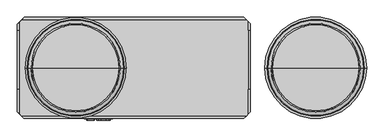
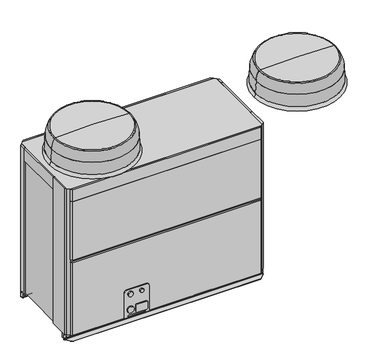
"""IFC4 building model written with IfcOpenShell, lengths in millimetres: proxy geometry, PURY-P168-288_YSJMU_Heat_Recovery_460V : PURY-P192YSJMU-A(-BS)_460V."""

from ifc_helpers import new_model, si_unit, point, frame, frame_2d, origin, place, context, project, spatial, polyline, circle_curve, ellipse_curve, trimmed, segment, composite_curve, outline, extrude, source, transform, mapped, element, save
from ifc_brep_helpers import plane_surface, cylinder_surface, revolved_surface, advanced_brep


def mechanical_equipment_7c6ddfd4(model_context):
    return source(origin(), model_context, "Body", "SolidModel", [
        advanced_brep(
        [(1130.4156536, 0.0, 1550.0000157), (1851.6603464, 0.0, 1550.0000157), (1491.038, 0.0, 1550.0000157), (1156.2569245, 0.0, 1635.7196156), (1825.8190755, 0.0, 1635.7196156), (1165.4260831, 0.0, 1640.2981249), (1816.6499169, 0.0, 1640.2981249), (1491.038, 0.0, 1649.794168)],
        [
            (0, 1, circle_curve(frame((1491.038, 0.0, 1550.0000157), z_axis=(0.0, 0.0, -1.0), x_axis=(1.0, 0.0, 0.0)), 360.6223464)),
            (1, 2),
            (2, 0),
            (1, 0, circle_curve(frame((1491.038, 0.0, 1550.0000157), z_axis=(0.0, 0.0, -1.0), x_axis=(1.0, 0.0, 0.0)), 360.6223464)),
            (3, 4, circle_curve(frame((1491.038, 0.0, 1635.7196156), z_axis=(0.0, 0.0, -1.0), x_axis=(1.0, 0.0, 0.0)), 334.7810755)),
            (4, 1, circle_curve(frame((1667.7568175, 0.0, 1541.3148332), z_axis=(0.0, 1.0, 0.0), x_axis=(1.0, 0.0, 0.0)), 184.1085015)),
            (0, 3, circle_curve(frame((1314.3191825, 0.0, 1541.3148332), z_axis=(0.0, 1.0, 0.0), x_axis=(-1.0, 0.0, 0.0)), 184.1085015)),
            (4, 3, circle_curve(frame((1491.038, 0.0, 1635.7196156), z_axis=(0.0, 0.0, -1.0), x_axis=(1.0, 0.0, 0.0)), 334.7810755)),
            (5, 6, circle_curve(frame((1491.038, 0.0, 1640.2981249), z_axis=(0.0, 0.0, -1.0), x_axis=(1.0, 0.0, 0.0)), 325.6119169)),
            (6, 4, circle_curve(frame((1816.6499169, 0.0, 1628.8275558), z_axis=(0.0, 1.0, 0.0), x_axis=(1.0, 0.0, 0.0)), 11.4705691)),
            (3, 5, circle_curve(frame((1165.4260831, 0.0, 1628.8275558), z_axis=(0.0, 1.0, 0.0), x_axis=(-1.0, 0.0, 0.0)), 11.4705691)),
            (6, 5, circle_curve(frame((1491.038, 0.0, 1640.2981249), z_axis=(0.0, 0.0, -1.0), x_axis=(1.0, 0.0, 0.0)), 325.6119169)),
            (7, 6, circle_curve(frame((1491.038, 0.0, -3937.4433334), z_axis=(0.0, 1.0, 0.0), x_axis=(1.0, 0.0, 0.0)), 5587.2375013)),
            (5, 7, circle_curve(frame((1491.038, 0.0, -3937.4433334), z_axis=(0.0, 1.0, 0.0), x_axis=(-1.0, 0.0, 0.0)), 5587.2375013)),
        ],
        [
            plane_surface(frame((1491.038, 0.0, 1550.0000157), z_axis=(0.0, 0.0, -1.0), x_axis=(1.0, 0.0, 0.0))),
            revolved_surface(trimmed(ellipse_curve(frame((1667.7568175, 0.0, 1541.3148332), z_axis=(0.0, -1.0, 0.0), x_axis=(1.0, 0.0, 0.0)), 184.1085015, 184.1085015), [point((1851.6603464, 0.0, 1550.0000157))], [point((1825.8190755, 0.0, 1635.7196156))], True, "CARTESIAN"), (1491.038, 0.0, 1605.0), (0.0, 0.0, 1.0)),
            revolved_surface(trimmed(ellipse_curve(frame((1816.6499169, 0.0, 1628.8275558), z_axis=(0.0, -1.0, 0.0), x_axis=(1.0, 0.0, 0.0)), 11.4705691, 11.4705691), [point((1825.8190755, 0.0, 1635.7196156))], [point((1816.6499169, 0.0, 1640.2981249))], True, "CARTESIAN"), (1491.038, 0.0, 1605.0), (0.0, 0.0, 1.0)),
            revolved_surface(trimmed(ellipse_curve(frame((1491.038, 0.0, -3937.4433334), z_axis=(0.0, -1.0, 0.0), x_axis=(1.0, 0.0, 0.0)), 5587.2375013, 5587.2375013), [point((1816.6499169, 0.0, 1640.2981249))], [point((1491.038, 0.0, 1649.794168))], True, "CARTESIAN"), (1491.038, 0.0, 1605.0), (0.0, 0.0, 1.0)),
        ],
        [
            (0, [[1, 2, 3]]),
            (0, [[4, -3, -2]]),
            (1, [[5, 6, -1, 7]]),
            (1, [[8, -7, -4, -6]]),
            (2, [[9, 10, -5, 11]]),
            (2, [[12, -11, -8, -10]]),
            (3, [[13, -9, 14]]),
            (3, [[-14, -12, -13]]),
        ],
    ),
        advanced_brep(
        [(1108.9881528, 0.0, 1410.0), (1873.0878472, 0.0, 1410.0), (1491.038, 0.0, 1410.0), (1125.5531583, 0.0, 1438.6914312), (1856.5228417, 0.0, 1438.6914312), (1130.4129453, 0.0, 1550.0000157), (1851.6630547, 0.0, 1550.0000157), (1491.038, 0.0, 1550.0000157)],
        [
            (0, 1, circle_curve(frame((1491.038, 0.0, 1410.0), z_axis=(0.0, 0.0, -1.0), x_axis=(1.0, 0.0, 0.0)), 382.0498472)),
            (1, 2),
            (2, 0),
            (1, 0, circle_curve(frame((1491.038, 0.0, 1410.0), z_axis=(0.0, 0.0, -1.0), x_axis=(1.0, 0.0, 0.0)), 382.0498472)),
            (3, 4, circle_curve(frame((1491.038, 0.0, 1438.6914312), z_axis=(0.0, 0.0, -1.0), x_axis=(1.0, 0.0, 0.0)), 365.4848417)),
            (4, 1, circle_curve(frame((1877.2748091, 0.0, 1431.5449644), z_axis=(0.0, -1.0, 0.0), x_axis=(1.0, 0.0, 0.0)), 21.9480327)),
            (0, 3, circle_curve(frame((1104.8011909, 0.0, 1431.5449644), z_axis=(0.0, -1.0, 0.0), x_axis=(-1.0, 0.0, 0.0)), 21.9480327)),
            (4, 3, circle_curve(frame((1491.038, 0.0, 1438.6914312), z_axis=(0.0, 0.0, -1.0), x_axis=(1.0, 0.0, 0.0)), 365.4848417)),
            (5, 6, circle_curve(frame((1491.038, 0.0, 1550.0000157), z_axis=(0.0, 0.0, -1.0), x_axis=(1.0, 0.0, 0.0)), 360.6250547)),
            (6, 4),
            (3, 5),
            (6, 5, circle_curve(frame((1491.038, 0.0, 1550.0000157), z_axis=(0.0, 0.0, -1.0), x_axis=(1.0, 0.0, 0.0)), 360.6250547)),
            (7, 6),
            (5, 7),
        ],
        [
            plane_surface(frame((1491.038, 0.0, 1410.0), z_axis=(0.0, 0.0, -1.0), x_axis=(1.0, 0.0, 0.0))),
            revolved_surface(trimmed(ellipse_curve(frame((1877.2748091, 0.0, 1431.5449644), z_axis=(0.0, 1.0, 0.0), x_axis=(1.0, 0.0, 0.0)), 21.9480327, 21.9480327), [point((1873.0878472, 0.0, 1410.0))], [point((1856.5228417, 0.0, 1438.6914312))], True, "CARTESIAN"), (1491.038, 0.0, 1470.0), (0.0, 0.0, 1.0)),
            revolved_surface(polyline([(1856.5228417, 0.0, 1438.6914312), (1851.6630547, 0.0, 1550.0000157)]), (1491.038, 0.0, 1470.0), (0.0, 0.0, 1.0)),
            plane_surface(frame((1491.038, 0.0, 1550.0000157), z_axis=(0.0, 0.0, 1.0), x_axis=(1.0, 0.0, 0.0))),
        ],
        [
            (0, [[1, 2, 3]]),
            (0, [[4, -3, -2]]),
            (1, [[5, 6, -1, 7]]),
            (1, [[8, -7, -4, -6]]),
            (2, [[9, 10, -5, 11]]),
            (2, [[12, -11, -8, -10]]),
            (3, [[13, -9, 14]]),
            (3, [[-14, -12, -13]]),
        ],
    ),
        extrude(outline(composite_curve([segment(trimmed(circle_curve(frame_2d((148.5853631, -142.3882489)), 9.9920268), [point((158.5773899, -142.3882489))], [point((148.5853631, -152.3802757))], False, "CARTESIAN"), True, "CONTINUOUS"), segment(polyline([(148.5853631, -152.3802757), (96.5694168, -152.3802757)]), True, "CONTINUOUS"), segment(trimmed(circle_curve(frame_2d((96.5694168, -142.3882489)), 9.9920268), [point((96.5694168, -152.3802757))], [point((86.5773899, -142.3882489))], False, "CARTESIAN"), True, "CONTINUOUS"), segment(polyline([(86.5773899, -142.3882489), (86.5773899, -60.3723026)]), True, "CONTINUOUS"), segment(trimmed(circle_curve(frame_2d((96.5694168, -60.3723026)), 9.9920268), [point((86.5773899, -60.3723026))], [point((96.5694168, -50.3802757))], False, "CARTESIAN"), True, "CONTINUOUS"), segment(polyline([(96.5694168, -50.3802757), (148.5853631, -50.3802757)]), True, "CONTINUOUS"), segment(trimmed(circle_curve(frame_2d((148.5853631, -60.3723026)), 9.9920268), [point((148.5853631, -50.3802757))], [point((158.5773899, -60.3723026))], False, "CARTESIAN"), True, "CONTINUOUS"), segment(polyline([(158.5773899, -60.3723026), (158.5773899, -142.3882489)]), True, "CONTINUOUS")], self_intersect=False)), frame((0.0, -397.2710787, 0.0), z_axis=(0.0, 1.0, 0.0), x_axis=(0.0, 0.0, 1.0)), (0.0, 0.0, 1.0), 12.5),
        extrude(outline(composite_curve([segment(trimmed(circle_curve(frame_2d((292.0295314, -55.1286698)), 21.9704686), [point((292.0295314, -33.1582012))], [point((314.0, -55.1286698))], False, "CARTESIAN"), True, "CONTINUOUS"), segment(polyline([(314.0, -55.1286698), (314.0, -226.9915314)]), True, "CONTINUOUS"), segment(trimmed(circle_curve(frame_2d((292.0295314, -226.9915314)), 21.9704686), [point((314.0, -226.9915314))], [point((292.0295314, -248.962))], False, "CARTESIAN"), True, "CONTINUOUS"), segment(polyline([(292.0295314, -248.962), (54.0, -248.962), (54.0, -33.1582012), (292.0295314, -33.1582012)]), True, "CONTINUOUS")], self_intersect=False), holes=[composite_curve([segment(trimmed(circle_curve(frame_2d((66.0219764, -74.4132816)), 7.4940201), [point((73.5159966, -74.4132816))], [point((58.5279563, -74.4132816))], True, "CARTESIAN"), True, "CONTINUOUS"), segment(polyline([(58.5279563, -74.4132816), (58.5279563, -209.3056439)]), True, "CONTINUOUS"), segment(trimmed(circle_curve(frame_2d((66.0219764, -209.3056439)), 7.4940201), [point((58.5279563, -209.3056439))], [point((73.5159966, -209.3056439))], True, "CARTESIAN"), True, "CONTINUOUS"), segment(polyline([(73.5159966, -209.3056439), (73.5159966, -74.4132816)]), True, "CONTINUOUS")], self_intersect=False)]), frame((0.0, -384.7710787, 0.0), z_axis=(0.0, 1.0, 0.0), x_axis=(0.0, 0.0, 1.0)), (0.0, 0.0, 1.0), 4.7710787),
        extrude(outline(composite_curve([segment(trimmed(circle_curve(frame_2d((272.5206481, -199.3802757)), 22.225), [point((272.5206481, -221.6052757))], [point((272.5206481, -177.1552757))], False, "CARTESIAN"), True, "CONTINUOUS"), segment(trimmed(circle_curve(frame_2d((272.5206481, -199.3802757)), 22.225), [point((272.5206481, -177.1552757))], [point((272.5206481, -221.6052757))], False, "CARTESIAN"), True, "CONTINUOUS")], self_intersect=False)), frame((0.0, -397.2710787, 0.0), z_axis=(0.0, 1.0, 0.0), x_axis=(0.0, 0.0, 1.0)), (0.0, 0.0, 1.0), 12.5),
        extrude(outline(composite_curve([segment(trimmed(circle_curve(frame_2d((272.5206481, -101.3802757)), 17.0), [point((272.5206481, -118.3802757))], [point((272.5206481, -84.3802757))], False, "CARTESIAN"), True, "CONTINUOUS"), segment(trimmed(circle_curve(frame_2d((272.5206481, -101.3802757)), 17.0), [point((272.5206481, -84.3802757))], [point((272.5206481, -118.3802757))], False, "CARTESIAN"), True, "CONTINUOUS")], self_intersect=False)), frame((0.0, -397.2710787, 0.0), z_axis=(0.0, 1.0, 0.0), x_axis=(0.0, 0.0, 1.0)), (0.0, 0.0, 1.0), 12.5),
        extrude(outline(composite_curve([segment(trimmed(circle_curve(frame_2d((127.8409633, -199.3802757)), 28.575), [point((127.8409633, -227.9552757))], [point((127.8409633, -170.8052757))], False, "CARTESIAN"), True, "CONTINUOUS"), segment(trimmed(circle_curve(frame_2d((127.8409633, -199.3802757)), 28.575), [point((127.8409633, -170.8052757))], [point((127.8409633, -227.9552757))], False, "CARTESIAN"), True, "CONTINUOUS")], self_intersect=False)), frame((0.0, -397.2710787, 0.0), z_axis=(0.0, 1.0, 0.0), x_axis=(0.0, 0.0, 1.0)), (0.0, 0.0, 1.0), 12.5),
        extrude(outline(polyline([(1001.038, 284.0), (985.038, 284.0), (985.038, 346.9999976), (1001.038, 330.9999976), (1001.038, 284.0)])), frame((0.0, 0.0, 54.0), z_axis=(0.0, 0.0, 1.0), x_axis=(1.0, 0.0, 0.0)), (0.0, 0.0, 1.0), 1356.0),
        extrude(outline(polyline([(985.038, -164.0), (1001.038, -164.0), (1001.038, -331.000002), (985.038, -347.000002), (985.038, -164.0)])), frame((0.0, 0.0, 54.0), z_axis=(0.0, 0.0, 1.0), x_axis=(1.0, 0.0, 0.0)), (0.0, 0.0, 1.0), 1356.0),
        extrude(outline(polyline([(932.5551598, 364.0), (932.5551598, 380.0), (952.0379976, 380.0), (968.0379976, 364.0), (932.5551598, 364.0)])), frame((0.0, 0.0, 54.0), z_axis=(0.0, 0.0, 1.0), x_axis=(1.0, 0.0, 0.0)), (0.0, 0.0, 1.0), 1245.8),
        extrude(outline(polyline([(-670.129169, 380.0), (-670.129169, 364.0), (-714.5495072, 364.0), (-698.5495072, 380.0), (-670.129169, 380.0)])), frame((0.0, 0.0, 54.0), z_axis=(0.0, 0.0, 1.0), x_axis=(1.0, 0.0, 0.0)), (0.0, 0.0, 1.0), 1245.8),
        extrude(outline(polyline([(968.0379976, 364.0), (-714.5495072, 364.0), (-698.5495072, 380.0), (952.0379976, 380.0), (968.0379976, 364.0)])), frame((0.0, 0.0, 1299.8), z_axis=(0.0, 0.0, 1.0), x_axis=(1.0, 0.0, 0.0)), (0.0, 0.0, 1.0), 110.2),
        extrude(outline(polyline([(952.038002, -380.0), (-699.9620129, -380.0), (-715.9620129, -364.0), (968.038002, -364.0), (952.038002, -380.0)])), frame((0.0, 0.0, 1299.8), z_axis=(0.0, 0.0, 1.0), x_axis=(1.0, 0.0, 0.0)), (0.0, 0.0, 1.0), 110.2),
        extrude(outline(polyline([(-715.9620129, -364.0), (968.038002, -364.0), (952.038002, -380.0), (-699.9620129, -380.0), (-715.9620129, -364.0)])), frame((0.0, 0.0, 755.5000076), z_axis=(0.0, 0.0, 1.0), x_axis=(1.0, 0.0, 0.0)), (0.0, 0.0, 1.0), 544.2999924),
        extrude(outline(polyline([(-732.962, -347.0000129), (-732.962, 345.5875072), (-714.5495072, 364.0), (968.0379976, 364.0), (985.038, 346.9999976), (985.038, -347.000002), (968.038002, -364.0), (-715.9620129, -364.0), (-732.962, -347.0000129)])), frame((0.0, 0.0, 54.0), z_axis=(0.0, 0.0, 1.0), x_axis=(1.0, 0.0, 0.0)), (0.0, 0.0, 1.0), 1356.0),
        extrude(outline(polyline([(-732.962, 284.0), (-748.962, 284.0), (-748.962, 329.5875072), (-732.962, 345.5875072), (-732.962, 284.0)])), frame((0.0, 0.0, 54.0), z_axis=(0.0, 0.0, 1.0), x_axis=(1.0, 0.0, 0.0)), (0.0, 0.0, 1.0), 1356.0),
        extrude(outline(polyline([(-748.962, -164.0), (-732.962, -164.0), (-732.962, -347.0000129), (-748.962, -331.0000129), (-748.962, -164.0)])), frame((0.0, 0.0, 54.0), z_axis=(0.0, 0.0, 1.0), x_axis=(1.0, 0.0, 0.0)), (0.0, 0.0, 1.0), 1356.0),
        extrude(outline(polyline([(-715.9620129, -364.0), (968.038002, -364.0), (952.038002, -380.0), (-699.9620129, -380.0), (-715.9620129, -364.0)])), frame((0.0, 0.0, 54.0), z_axis=(0.0, 0.0, 1.0), x_axis=(1.0, 0.0, 0.0)), (0.0, 0.0, 1.0), 678.5000074),
        extrude(outline(polyline([(161.038, 364.0), (161.038, 380.0), (932.5551598, 380.0), (932.5551598, 364.0), (161.038, 364.0)])), frame((0.0, 0.0, 54.0), z_axis=(0.0, 0.0, 1.0), x_axis=(1.0, 0.0, 0.0)), (0.0, 0.0, 1.0), 1245.8),
        extrude(outline(polyline([(161.038, 339.0), (141.038, 339.0), (141.038, 380.0), (161.038, 380.0), (161.038, 339.0)])), frame((0.0, 0.0, 54.0), z_axis=(0.0, 0.0, 1.0), x_axis=(1.0, 0.0, 0.0)), (0.0, 0.0, 1.0), 1245.8),
        extrude(outline(polyline([(111.038, 339.0), (91.038, 339.0), (91.038, 380.0), (111.038, 380.0), (111.038, 339.0)])), frame((0.0, 0.0, 54.0), z_axis=(0.0, 0.0, 1.0), x_axis=(1.0, 0.0, 0.0)), (0.0, 0.0, 1.0), 1245.8),
        advanced_brep(
        [(-672.0843464, 0.0, 1550.0000157), (49.1603464, 0.0, 1550.0000157), (-311.462, 0.0, 1550.0000157), (-646.2430755, 0.0, 1635.7196156), (23.3190755, 0.0, 1635.7196156), (-637.0739169, 0.0, 1640.2981249), (14.1499169, 0.0, 1640.2981249), (-311.462, 0.0, 1649.7941679)],
        [
            (0, 1, circle_curve(frame((-311.462, 0.0, 1550.0000157), z_axis=(0.0, 0.0, -1.0), x_axis=(1.0, 0.0, 0.0)), 360.6223464)),
            (1, 2),
            (2, 0),
            (1, 0, circle_curve(frame((-311.462, 0.0, 1550.0000157), z_axis=(0.0, 0.0, -1.0), x_axis=(1.0, 0.0, 0.0)), 360.6223464)),
            (3, 4, circle_curve(frame((-311.462, 0.0, 1635.7196156), z_axis=(0.0, 0.0, -1.0), x_axis=(1.0, 0.0, 0.0)), 334.7810755)),
            (4, 1, circle_curve(frame((-134.7431825, 0.0, 1541.3148332), z_axis=(0.0, 1.0, 0.0), x_axis=(1.0, 0.0, 0.0)), 184.1085015)),
            (0, 3, circle_curve(frame((-488.1808175, 0.0, 1541.3148332), z_axis=(0.0, 1.0, 0.0), x_axis=(-1.0, 0.0, 0.0)), 184.1085015)),
            (4, 3, circle_curve(frame((-311.462, 0.0, 1635.7196156), z_axis=(0.0, 0.0, -1.0), x_axis=(1.0, 0.0, 0.0)), 334.7810755)),
            (5, 6, circle_curve(frame((-311.462, 0.0, 1640.2981249), z_axis=(0.0, 0.0, -1.0), x_axis=(1.0, 0.0, 0.0)), 325.6119169)),
            (6, 4, circle_curve(frame((14.1499169, 0.0, 1628.8275558), z_axis=(0.0, 1.0, 0.0), x_axis=(1.0, 0.0, 0.0)), 11.4705691)),
            (3, 5, circle_curve(frame((-637.0739169, 0.0, 1628.8275558), z_axis=(0.0, 1.0, 0.0), x_axis=(-1.0, 0.0, 0.0)), 11.4705691)),
            (6, 5, circle_curve(frame((-311.462, 0.0, 1640.2981249), z_axis=(0.0, 0.0, -1.0), x_axis=(1.0, 0.0, 0.0)), 325.6119169)),
            (7, 6, circle_curve(frame((-311.462, 0.0, -3937.4433334), z_axis=(0.0, 1.0, 0.0), x_axis=(1.0, 0.0, 0.0)), 5587.2375013)),
            (5, 7, circle_curve(frame((-311.462, 0.0, -3937.4433334), z_axis=(0.0, 1.0, 0.0), x_axis=(-1.0, 0.0, 0.0)), 5587.2375013)),
        ],
        [
            plane_surface(frame((-311.462, 0.0, 1550.0000157), z_axis=(0.0, 0.0, -1.0), x_axis=(1.0, 0.0, 0.0))),
            revolved_surface(trimmed(ellipse_curve(frame((-134.7431825, 0.0, 1541.3148332), z_axis=(0.0, -1.0, 0.0), x_axis=(1.0, 0.0, 0.0)), 184.1085015, 184.1085015), [point((49.1603464, 0.0, 1550.0000157))], [point((23.3190755, 0.0, 1635.7196156))], True, "CARTESIAN"), (-311.462, 0.0, 1605.0), (0.0, 0.0, 1.0)),
            revolved_surface(trimmed(ellipse_curve(frame((14.1499169, 0.0, 1628.8275558), z_axis=(0.0, -1.0, 0.0), x_axis=(1.0, 0.0, 0.0)), 11.4705691, 11.4705691), [point((23.3190755, 0.0, 1635.7196156))], [point((14.1499169, 0.0, 1640.2981249))], True, "CARTESIAN"), (-311.462, 0.0, 1605.0), (0.0, 0.0, 1.0)),
            revolved_surface(trimmed(ellipse_curve(frame((-311.462, 0.0, -3937.4433334), z_axis=(0.0, -1.0, 0.0), x_axis=(1.0, 0.0, 0.0)), 5587.2375013, 5587.2375013), [point((14.1499169, 0.0, 1640.2981249))], [point((-311.462, 0.0, 1649.7941679))], True, "CARTESIAN"), (-311.462, 0.0, 1605.0), (0.0, 0.0, 1.0)),
        ],
        [
            (0, [[1, 2, 3]]),
            (0, [[4, -3, -2]]),
            (1, [[5, 6, -1, 7]]),
            (1, [[8, -7, -4, -6]]),
            (2, [[9, 10, -5, 11]]),
            (2, [[12, -11, -8, -10]]),
            (3, [[13, -9, 14]]),
            (3, [[-14, -12, -13]]),
        ],
    ),
        advanced_brep(
        [(-693.5118472, 0.0, 1410.0), (70.5878472, 0.0, 1410.0), (-311.462, 0.0, 1410.0), (-676.9468417, 0.0, 1438.6914312), (54.0228417, 0.0, 1438.6914312), (-672.0870547, 0.0, 1550.0000157), (49.1630547, 0.0, 1550.0000157), (-311.462, 0.0, 1550.0000157)],
        [
            (0, 1, circle_curve(frame((-311.462, 0.0, 1410.0), z_axis=(0.0, 0.0, -1.0), x_axis=(1.0, 0.0, 0.0)), 382.0498472)),
            (1, 2),
            (2, 0),
            (1, 0, circle_curve(frame((-311.462, 0.0, 1410.0), z_axis=(0.0, 0.0, -1.0), x_axis=(1.0, 0.0, 0.0)), 382.0498472)),
            (3, 4, circle_curve(frame((-311.462, 0.0, 1438.6914312), z_axis=(0.0, 0.0, -1.0), x_axis=(1.0, 0.0, 0.0)), 365.4848417)),
            (4, 1, circle_curve(frame((74.7748091, 0.0, 1431.5449644), z_axis=(0.0, -1.0, 0.0), x_axis=(1.0, 0.0, 0.0)), 21.9480327)),
            (0, 3, circle_curve(frame((-697.6988091, 0.0, 1431.5449644), z_axis=(0.0, -1.0, 0.0), x_axis=(-1.0, 0.0, 0.0)), 21.9480327)),
            (4, 3, circle_curve(frame((-311.462, 0.0, 1438.6914312), z_axis=(0.0, 0.0, -1.0), x_axis=(1.0, 0.0, 0.0)), 365.4848417)),
            (5, 6, circle_curve(frame((-311.462, 0.0, 1550.0000157), z_axis=(0.0, 0.0, -1.0), x_axis=(1.0, 0.0, 0.0)), 360.6250547)),
            (6, 4),
            (3, 5),
            (6, 5, circle_curve(frame((-311.462, 0.0, 1550.0000157), z_axis=(0.0, 0.0, -1.0), x_axis=(1.0, 0.0, 0.0)), 360.6250547)),
            (7, 6),
            (5, 7),
        ],
        [
            plane_surface(frame((-311.462, 0.0, 1410.0), z_axis=(0.0, 0.0, -1.0), x_axis=(1.0, 0.0, 0.0))),
            revolved_surface(trimmed(ellipse_curve(frame((74.7748091, 0.0, 1431.5449644), z_axis=(0.0, 1.0, 0.0), x_axis=(1.0, 0.0, 0.0)), 21.9480327, 21.9480327), [point((70.5878472, 0.0, 1410.0))], [point((54.0228417, 0.0, 1438.6914312))], True, "CARTESIAN"), (-311.462, 0.0, 1470.0), (0.0, 0.0, 1.0)),
            revolved_surface(polyline([(54.0228417, 0.0, 1438.6914312), (49.1630547, 0.0, 1550.0000157)]), (-311.462, 0.0, 1470.0), (0.0, 0.0, 1.0)),
            plane_surface(frame((-311.462, 0.0, 1550.0000157), z_axis=(0.0, 0.0, 1.0), x_axis=(1.0, 0.0, 0.0))),
        ],
        [
            (0, [[1, 2, 3]]),
            (0, [[4, -3, -2]]),
            (1, [[5, 6, -1, 7]]),
            (1, [[8, -7, -4, -6]]),
            (2, [[9, 10, -5, 11]]),
            (2, [[12, -11, -8, -10]]),
            (3, [[13, -9, 14]]),
            (3, [[-14, -12, -13]]),
        ],
    ),
        extrude(outline(polyline([(-670.129169, 364.0), (-670.129169, 380.0), (91.038, 380.0), (91.038, 364.0), (-670.129169, 364.0)])), frame((0.0, 0.0, 54.0), z_axis=(0.0, 0.0, 1.0), x_axis=(1.0, 0.0, 0.0)), (0.0, 0.0, 1.0), 1245.8),
        advanced_brep(
        [(1001.038, 330.9999976, 2.3), (1001.038, 330.9999976, 0.0), (952.0379976, 380.0, 0.0), (952.0379976, 380.0, 2.3), (-748.962, 329.5875072, 0.0), (-748.962, 329.5875072, 2.3), (-698.5495072, 380.0, 2.3), (-698.5495072, 380.0, 0.0), (1001.038, 329.5875072, 2.3), (1001.038, 324.5875071, 7.3000001), (1001.038, 324.5875071, 11.7000001), (1001.038, 325.5875071, 12.7000001), (1001.038, 327.5875072, 12.7000001), (1001.038, 327.5875072, 47.3000005), (1001.038, 325.5875071, 47.3000005), (1001.038, 324.5875071, 48.3000005), (1001.038, 324.5875071, 50.0000004), (1001.038, 320.5875077, 53.9999997), (1001.038, 299.5875069, 53.9999997), (1001.038, 299.5875069, 14.0000001), (1001.038, 304.5875069, 9.0000001), (1001.038, 322.2875071, 9.0000001), (1001.038, 322.2875071, 7.3000001), (1001.038, 329.5875072, 0.0), (-748.962, 322.2875071, 7.3000001), (-748.962, 322.2875071, 9.0000001), (-748.962, 304.5875069, 9.0000001), (-748.962, 299.5875069, 14.0000001), (-748.962, 299.5875069, 53.9999997), (-748.962, 320.5875077, 53.9999997), (-748.962, 324.5875071, 50.0000004), (-748.962, 324.5875071, 48.3000005), (-748.962, 325.5875071, 47.3000005), (-748.962, 327.5875072, 47.3000005), (-748.962, 327.5875072, 12.7000001), (-748.962, 325.5875071, 12.7000001), (-748.962, 324.5875071, 11.7000001), (-748.962, 324.5875071, 7.3000001), (972.288009, 327.5875072, 45.0000005), (930.7880086, 327.5875072, 45.0000005), (924.7880085, 327.5875072, 39.0000004), (924.7880085, 327.5875072, 21.0000002), (930.7880086, 327.5875072, 15.0000002), (972.288009, 327.5875072, 15.0000002), (978.2880091, 327.5875072, 21.0000002), (978.2880091, 327.5875072, 39.0000004), (-720.9619997, 327.5875072, 45.0000005), (-726.9619998, 327.5875072, 39.0000004), (-726.9619998, 327.5875072, 21.0000002), (-720.9619997, 327.5875072, 15.0000002), (-679.4619993, 327.5875072, 15.0000002), (-673.4619992, 327.5875072, 21.0000002), (-673.4619992, 327.5875072, 39.0000004), (-679.4619993, 327.5875072, 45.0000005), (930.7880086, 299.5875069, 45.0000005), (972.288009, 299.5875069, 45.0000005), (978.2880091, 299.5875069, 39.0000004), (978.2880091, 299.5875069, 21.0000002), (972.288009, 299.5875069, 15.0000002), (930.7880086, 299.5875069, 15.0000002), (924.7880085, 299.5875069, 21.0000002), (924.7880085, 299.5875069, 39.0000004), (-726.9619998, 299.5875069, 39.0000004), (-720.9619997, 299.5875069, 45.0000005), (-679.4619993, 299.5875069, 45.0000005), (-673.4619992, 299.5875069, 39.0000004), (-673.4619992, 299.5875069, 21.0000002), (-679.4619993, 299.5875069, 15.0000002), (-720.9619997, 299.5875069, 15.0000002), (-726.9619998, 299.5875069, 21.0000002)],
        [
            (0, 1),
            (1, 2),
            (2, 3),
            (3, 0),
            (4, 5),
            (5, 6),
            (6, 7),
            (7, 4),
            (8, 9, circle_curve(frame((1001.038, 329.5875072, 7.3000001), z_axis=(-1.0, 0.0, 0.0), x_axis=(0.0, 1.0, 0.0)), 5.0000001)),
            (9, 10),
            (10, 11, circle_curve(frame((1001.038, 325.5875071, 11.7000001), z_axis=(-1.0, 0.0, 0.0), x_axis=(0.0, 1.0, 0.0)), 1.0)),
            (11, 12),
            (12, 13),
            (13, 14),
            (14, 15, circle_curve(frame((1001.038, 325.5875071, 48.3000005), z_axis=(-1.0, 0.0, 0.0), x_axis=(0.0, 1.0, 0.0)), 1.0)),
            (15, 16),
            (16, 17, circle_curve(frame((1001.038, 320.5875077, 50.0000004), z_axis=(1.0, 0.0, 0.0), x_axis=(0.0, 1.0, 0.0)), 3.9999994)),
            (17, 18),
            (18, 19),
            (19, 20, circle_curve(frame((1001.038, 304.5875069, 14.0000001), z_axis=(1.0, 0.0, 0.0), x_axis=(0.0, 1.0, 0.0)), 5.0000001)),
            (20, 21),
            (21, 22),
            (22, 23, circle_curve(frame((1001.038, 329.5875072, 7.3000001), z_axis=(1.0, 0.0, 0.0), x_axis=(0.0, 1.0, 0.0)), 7.3000001)),
            (23, 1),
            (0, 8),
            (4, 24, circle_curve(frame((-748.962, 329.5875072, 7.3000001), z_axis=(-1.0, 0.0, 0.0), x_axis=(0.0, 1.0, 0.0)), 7.3000001)),
            (24, 25),
            (25, 26),
            (26, 27, circle_curve(frame((-748.962, 304.5875069, 14.0000001), z_axis=(-1.0, 0.0, 0.0), x_axis=(0.0, 1.0, 0.0)), 5.0000001)),
            (27, 28),
            (28, 29),
            (29, 30, circle_curve(frame((-748.962, 320.5875077, 50.0000004), z_axis=(-1.0, 0.0, 0.0), x_axis=(0.0, 1.0, 0.0)), 3.9999994)),
            (30, 31),
            (31, 32, circle_curve(frame((-748.962, 325.5875071, 48.3000005), z_axis=(1.0, 0.0, 0.0), x_axis=(0.0, 1.0, 0.0)), 1.0)),
            (32, 33),
            (33, 34),
            (34, 35),
            (35, 36, circle_curve(frame((-748.962, 325.5875071, 11.7000001), z_axis=(1.0, 0.0, 0.0), x_axis=(0.0, 1.0, 0.0)), 1.0)),
            (36, 37),
            (37, 5, circle_curve(frame((-748.962, 329.5875072, 7.3000001), z_axis=(1.0, 0.0, 0.0), x_axis=(0.0, 1.0, 0.0)), 5.0000001)),
            (8, 5),
            (37, 9),
            (36, 10),
            (35, 11),
            (34, 12),
            (33, 13),
            (38, 39),
            (39, 40, circle_curve(frame((930.7880086, 327.5875072, 39.0000004), z_axis=(0.0, -1.0, 0.0), x_axis=(1.0, 0.0, 0.0)), 6.0000001)),
            (40, 41),
            (41, 42, circle_curve(frame((930.7880086, 327.5875072, 21.0000002), z_axis=(0.0, -1.0, 0.0), x_axis=(1.0, 0.0, 0.0)), 6.0000001)),
            (42, 43),
            (43, 44, circle_curve(frame((972.288009, 327.5875072, 21.0000002), z_axis=(0.0, -1.0, 0.0), x_axis=(1.0, 0.0, 0.0)), 6.0000001)),
            (44, 45),
            (45, 38, circle_curve(frame((972.288009, 327.5875072, 39.0000004), z_axis=(0.0, -1.0, 0.0), x_axis=(1.0, 0.0, 0.0)), 6.0000001)),
            (46, 47, circle_curve(frame((-720.9619997, 327.5875072, 39.0000004), z_axis=(0.0, -1.0, 0.0), x_axis=(1.0, 0.0, 0.0)), 6.0000001)),
            (47, 48),
            (48, 49, circle_curve(frame((-720.9619997, 327.5875072, 21.0000002), z_axis=(0.0, -1.0, 0.0), x_axis=(1.0, 0.0, 0.0)), 6.0000001)),
            (49, 50),
            (50, 51, circle_curve(frame((-679.4619993, 327.5875072, 21.0000002), z_axis=(0.0, -1.0, 0.0), x_axis=(1.0, 0.0, 0.0)), 6.0000001)),
            (51, 52),
            (52, 53, circle_curve(frame((-679.4619993, 327.5875072, 39.0000004), z_axis=(0.0, -1.0, 0.0), x_axis=(1.0, 0.0, 0.0)), 6.0000001)),
            (53, 46),
            (32, 14),
            (31, 15),
            (30, 16),
            (29, 17),
            (28, 18),
            (27, 19),
            (54, 55),
            (55, 56, circle_curve(frame((972.288009, 299.5875069, 39.0000004), z_axis=(0.0, 1.0, 0.0), x_axis=(1.0, 0.0, 0.0)), 6.0000001)),
            (56, 57),
            (57, 58, circle_curve(frame((972.288009, 299.5875069, 21.0000002), z_axis=(0.0, 1.0, 0.0), x_axis=(1.0, 0.0, 0.0)), 6.0000001)),
            (58, 59),
            (59, 60, circle_curve(frame((930.7880086, 299.5875069, 21.0000002), z_axis=(0.0, 1.0, 0.0), x_axis=(1.0, 0.0, 0.0)), 6.0000001)),
            (60, 61),
            (61, 54, circle_curve(frame((930.7880086, 299.5875069, 39.0000004), z_axis=(0.0, 1.0, 0.0), x_axis=(1.0, 0.0, 0.0)), 6.0000001)),
            (62, 63, circle_curve(frame((-720.9619997, 299.5875069, 39.0000004), z_axis=(0.0, 1.0, 0.0), x_axis=(1.0, 0.0, 0.0)), 6.0000001)),
            (63, 64),
            (64, 65, circle_curve(frame((-679.4619993, 299.5875069, 39.0000004), z_axis=(0.0, 1.0, 0.0), x_axis=(1.0, 0.0, 0.0)), 6.0000001)),
            (65, 66),
            (66, 67, circle_curve(frame((-679.4619993, 299.5875069, 21.0000002), z_axis=(0.0, 1.0, 0.0), x_axis=(1.0, 0.0, 0.0)), 6.0000001)),
            (67, 68),
            (68, 69, circle_curve(frame((-720.9619997, 299.5875069, 21.0000002), z_axis=(0.0, 1.0, 0.0), x_axis=(1.0, 0.0, 0.0)), 6.0000001)),
            (69, 62),
            (26, 20),
            (25, 21),
            (24, 22),
            (4, 23),
            (7, 2),
            (6, 3),
            (38, 55),
            (54, 39),
            (61, 40),
            (60, 41),
            (59, 42),
            (58, 43),
            (57, 44),
            (56, 45),
            (46, 63),
            (62, 47),
            (69, 48),
            (68, 49),
            (67, 50),
            (66, 51),
            (65, 52),
            (64, 53),
        ],
        [
            plane_surface(frame((952.0379976, 380.0, 1410.0), z_axis=(0.7071067811865354, 0.7071067811865598, 0.0), x_axis=(0.0, 0.0, -1.0))),
            plane_surface(frame((-748.962, 329.5875072, 1410.0), z_axis=(-0.707106781186156, 0.7071067811869391, 0.0), x_axis=(0.0, 0.0, -1.0))),
            plane_surface(frame((1001.038, 334.5875072, 7.3000001), z_axis=(1.0, 0.0, 0.0), x_axis=(0.0, 0.0, -1.0))),
            plane_surface(frame((-748.962, 334.5875072, 7.3000001), z_axis=(-1.0, 0.0, 0.0), x_axis=(0.0, 0.0, 1.0))),
            revolved_surface(polyline([(-748.962, 334.5875073, 7.3000001), (1001.038, 334.5875073, 7.3000001)]), (-748.962, 329.5875072, 7.3000001), (-1.0, 0.0, 0.0)),
            plane_surface(frame((1001.038, 324.5875071, 7.3000001), z_axis=(0.0, 1.0, 0.0), x_axis=(-1.0, 0.0, 0.0))),
            revolved_surface(polyline([(-748.962, 326.5875071, 11.7000001), (1001.038, 326.5875071, 11.7000001)]), (-748.962, 325.5875071, 11.7000001), (-1.0, 0.0, 0.0)),
            plane_surface(frame((1001.038, 325.5875071, 12.7000001), z_axis=(0.0, 0.0, -1.0), x_axis=(-1.0, 0.0, 0.0))),
            plane_surface(frame((1001.038, 327.5875072, 12.7000001), z_axis=(0.0, 1.0, 0.0), x_axis=(-1.0, 0.0, 0.0))),
            plane_surface(frame((1001.038, 327.5875072, 47.3000005), z_axis=(0.0, 0.0, 1.0), x_axis=(-1.0, 0.0, 0.0))),
            revolved_surface(polyline([(-748.962, 326.5875071, 48.3000005), (1001.038, 326.5875071, 48.3000005)]), (-748.962, 325.5875071, 48.3000005), (-1.0, 0.0, 0.0)),
            plane_surface(frame((1001.038, 324.5875071, 48.3000005), z_axis=(0.0, 1.0, 0.0), x_axis=(-1.0, 0.0, 0.0))),
            cylinder_surface(frame((-748.962, 320.5875077, 50.0000004), z_axis=(1.0, 0.0, 0.0), x_axis=(0.0, 1.0, 0.0)), 3.9999994),
            plane_surface(frame((1001.038, 320.5875077, 53.9999997), z_axis=(0.0, 0.0, 1.0), x_axis=(-1.0, 0.0, 0.0))),
            plane_surface(frame((1001.038, 299.5875069, 53.9999997), z_axis=(0.0, -1.0, 0.0), x_axis=(-1.0, 0.0, 0.0))),
            cylinder_surface(frame((-748.962, 304.5875069, 14.0000001), z_axis=(1.0, 0.0, 0.0), x_axis=(0.0, 1.0, 0.0)), 5.0000001),
            plane_surface(frame((1001.038, 304.5875069, 9.0000001), z_axis=(0.0, 0.0, -1.0), x_axis=(-1.0, 0.0, 0.0))),
            plane_surface(frame((1001.038, 322.2875071, 9.0000001), z_axis=(0.0, -1.0, 0.0), x_axis=(-1.0, 0.0, 0.0))),
            cylinder_surface(frame((-748.962, 329.5875072, 7.3000001), z_axis=(1.0, 0.0, 0.0), x_axis=(0.0, 1.0, 0.0)), 7.3000001),
            plane_surface(frame((1001.038, 329.5875072, 0.0), z_axis=(0.0, 0.0, -1.0), x_axis=(-1.0, 0.0, 0.0))),
            plane_surface(frame((1001.038, 380.0, 0.0), z_axis=(0.0, 1.0, 0.0), x_axis=(-1.0, 0.0, 0.0))),
            plane_surface(frame((1001.038, 380.0, 2.3), z_axis=(0.0, 0.0, 1.0), x_axis=(-1.0, 0.0, 0.0))),
            plane_surface(frame((972.288009, -339.0, 45.0000005), z_axis=(0.0, 0.0, -1.0), x_axis=(0.0, 1.0, 0.0))),
            revolved_surface(polyline([(936.7880087, 299.5875069, 39.0000004), (936.7880087, 327.5875072, 39.0000004)]), (930.7880086, 339.0, 39.0000004), (0.0, -1.0, 0.0)),
            plane_surface(frame((924.7880085, -339.0, 39.0000004), z_axis=(1.0, 0.0, 0.0), x_axis=(0.0, 1.0, 0.0))),
            revolved_surface(polyline([(936.7880087, 299.5875069, 21.0000002), (936.7880087, 327.5875072, 21.0000002)]), (930.7880086, 339.0, 21.0000002), (0.0, -1.0, 0.0)),
            plane_surface(frame((930.7880086, -339.0, 15.0000002), z_axis=(0.0, 0.0, 1.0), x_axis=(0.0, 1.0, 0.0))),
            revolved_surface(polyline([(978.2880091, 299.5875069, 21.0000002), (978.2880091, 327.5875072, 21.0000002)]), (972.288009, 339.0, 21.0000002), (0.0, -1.0, 0.0)),
            plane_surface(frame((978.2880091, -339.0, 21.0000002), z_axis=(-1.0, 0.0, 0.0), x_axis=(0.0, 1.0, 0.0))),
            revolved_surface(polyline([(978.2880091, 299.5875069, 39.0000004), (978.2880091, 327.5875072, 39.0000004)]), (972.288009, 339.0, 39.0000004), (0.0, -1.0, 0.0)),
            revolved_surface(polyline([(-714.9619996, 299.5875069, 39.0000004), (-714.9619996, 327.5875072, 39.0000004)]), (-720.9619997, 0.0, 39.0000004), (0.0, -1.0, 0.0)),
            plane_surface(frame((-726.9619998, -339.0, 39.0000004), z_axis=(1.0, 0.0, 0.0), x_axis=(0.0, 1.0, 0.0))),
            revolved_surface(polyline([(-714.9619996, 299.5875069, 21.0000002), (-714.9619996, 327.5875072, 21.0000002)]), (-720.9619997, 0.0, 21.0000002), (0.0, -1.0, 0.0)),
            plane_surface(frame((-720.9619997, -339.0, 15.0000002), z_axis=(0.0, 0.0, 1.0), x_axis=(0.0, 1.0, 0.0))),
            revolved_surface(polyline([(-673.4619992, 299.5875069, 21.0000002), (-673.4619992, 327.5875072, 21.0000002)]), (-679.4619993, 0.0, 21.0000002), (0.0, -1.0, 0.0)),
            plane_surface(frame((-673.4619992, -339.0, 21.0000002), z_axis=(-1.0, 0.0, 0.0), x_axis=(0.0, 1.0, 0.0))),
            revolved_surface(polyline([(-673.4619992, 299.5875069, 39.0000004), (-673.4619992, 327.5875072, 39.0000004)]), (-679.4619993, 0.0, 39.0000004), (0.0, -1.0, 0.0)),
            plane_surface(frame((-679.4619993, -339.0, 45.0000005), z_axis=(0.0, 0.0, -1.0), x_axis=(0.0, 1.0, 0.0))),
        ],
        [
            (0, [[1, 2, 3, 4]]),
            (1, [[5, 6, 7, 8]]),
            (2, [[9, 10, 11, 12, 13, 14, 15, 16, 17, 18, 19, 20, 21, 22, 23, 24, -1, 25]]),
            (3, [[26, 27, 28, 29, 30, 31, 32, 33, 34, 35, 36, 37, 38, 39, 40, -5]]),
            (4, [[-9, 41, -40, 42]]),
            (5, [[-10, -42, -39, 43]]),
            (6, [[-11, -43, -38, 44]]),
            (7, [[-12, -44, -37, 45]]),
            (8, [[-13, -45, -36, 46], [47, 48, 49, 50, 51, 52, 53, 54], [55, 56, 57, 58, 59, 60, 61, 62]]),
            (9, [[-14, -46, -35, 63]]),
            (10, [[-15, -63, -34, 64]]),
            (11, [[-16, -64, -33, 65]]),
            (12, [[-17, -65, -32, 66]]),
            (13, [[-18, -66, -31, 67]]),
            (14, [[-19, -67, -30, 68], [69, 70, 71, 72, 73, 74, 75, 76], [77, 78, 79, 80, 81, 82, 83, 84]]),
            (15, [[-20, -68, -29, 85]]),
            (16, [[-21, -85, -28, 86]]),
            (17, [[-22, -86, -27, 87]]),
            (18, [[-23, -87, -26, 88]]),
            (19, [[-88, -8, 89, -2, -24]]),
            (20, [[-89, -7, 90, -3]]),
            (21, [[-41, -25, -4, -90, -6]]),
            (22, [[91, -69, 92, -47]]),
            (23, [[-92, -76, 93, -48]]),
            (24, [[-93, -75, 94, -49]]),
            (25, [[-94, -74, 95, -50]]),
            (26, [[-95, -73, 96, -51]]),
            (27, [[-96, -72, 97, -52]]),
            (28, [[-97, -71, 98, -53]]),
            (29, [[-91, -54, -98, -70]]),
            (30, [[99, -77, 100, -55]]),
            (31, [[-100, -84, 101, -56]]),
            (32, [[-101, -83, 102, -57]]),
            (33, [[-102, -82, 103, -58]]),
            (34, [[-103, -81, 104, -59]]),
            (35, [[-104, -80, 105, -60]]),
            (36, [[-105, -79, 106, -61]]),
            (37, [[-99, -62, -106, -78]]),
        ],
    ),
        advanced_brep(
        [(1001.038, -331.000002, 0.0), (1001.038, -331.000002, 2.3), (952.038002, -380.0, 2.3), (952.038002, -380.0, 0.0), (-748.962, -331.0000129, 2.3), (-748.962, -331.0000129, 0.0), (-699.9620129, -380.0, 0.0), (-699.9620129, -380.0, 2.3), (1001.038, -329.9000072, 0.0), (1001.038, -322.6000071, 7.3000001), (1001.038, -322.6000071, 9.0000001), (1001.038, -304.9000069, 9.0000001), (1001.038, -299.9000069, 14.0000001), (1001.038, -299.9000069, 53.9999997), (1001.038, -320.9000077, 53.9999997), (1001.038, -324.9000071, 50.0000004), (1001.038, -324.9000071, 48.3000005), (1001.038, -325.9000071, 47.3000005), (1001.038, -327.9000072, 47.3000005), (1001.038, -327.9000072, 12.7000001), (1001.038, -325.9000071, 12.7000001), (1001.038, -324.9000071, 11.7000001), (1001.038, -324.9000071, 7.3000001), (1001.038, -329.9000072, 2.3), (-748.962, -329.9000072, 2.3), (-748.962, -324.9000071, 7.3000001), (-748.962, -324.9000071, 11.7000001), (-748.962, -325.9000071, 12.7000001), (-748.962, -327.9000072, 12.7000001), (-748.962, -327.9000072, 47.3000005), (-748.962, -325.9000071, 47.3000005), (-748.962, -324.9000071, 48.3000005), (-748.962, -324.9000071, 50.0000004), (-748.962, -320.9000077, 53.9999997), (-748.962, -299.9000069, 53.9999997), (-748.962, -299.9000069, 14.0000001), (-748.962, -304.9000069, 9.0000001), (-748.962, -322.6000071, 9.0000001), (-748.962, -322.6000071, 7.3000001), (-748.962, -329.9000072, 0.0), (972.288009, -299.9000069, 45.0000005), (930.7880086, -299.9000069, 45.0000005), (924.7880085, -299.9000069, 39.0000004), (924.7880085, -299.9000069, 21.0000002), (930.7880086, -299.9000069, 15.0000002), (972.288009, -299.9000069, 15.0000002), (978.2880091, -299.9000069, 21.0000002), (978.2880091, -299.9000069, 39.0000004), (-720.9619997, -299.9000069, 45.0000005), (-726.9619998, -299.9000069, 39.0000004), (-726.9619998, -299.9000069, 21.0000002), (-720.9619997, -299.9000069, 15.0000002), (-679.4619993, -299.9000069, 15.0000002), (-673.4619992, -299.9000069, 21.0000002), (-673.4619992, -299.9000069, 39.0000004), (-679.4619993, -299.9000069, 45.0000005), (930.7880086, -327.9000072, 45.0000005), (972.288009, -327.9000072, 45.0000005), (978.2880091, -327.9000072, 39.0000004), (978.2880091, -327.9000072, 21.0000002), (972.288009, -327.9000072, 15.0000002), (930.7880086, -327.9000072, 15.0000002), (924.7880085, -327.9000072, 21.0000002), (924.7880085, -327.9000072, 39.0000004), (-726.9619998, -327.9000072, 39.0000004), (-720.9619997, -327.9000072, 45.0000005), (-679.4619993, -327.9000072, 45.0000005), (-673.4619992, -327.9000072, 39.0000004), (-673.4619992, -327.9000072, 21.0000002), (-679.4619993, -327.9000072, 15.0000002), (-720.9619997, -327.9000072, 15.0000002), (-726.9619998, -327.9000072, 21.0000002)],
        [
            (0, 1),
            (1, 2),
            (2, 3),
            (3, 0),
            (4, 5),
            (5, 6),
            (6, 7),
            (7, 4),
            (8, 9, circle_curve(frame((1001.038, -329.9000072, 7.3000001), z_axis=(1.0, 0.0, 0.0), x_axis=(0.0, 1.0, 0.0)), 7.3000001)),
            (9, 10),
            (10, 11),
            (11, 12, circle_curve(frame((1001.038, -304.9000069, 14.0000001), z_axis=(1.0, 0.0, 0.0), x_axis=(0.0, 1.0, 0.0)), 5.0000001)),
            (12, 13),
            (13, 14),
            (14, 15, circle_curve(frame((1001.038, -320.9000077, 50.0000004), z_axis=(1.0, 0.0, 0.0), x_axis=(0.0, 1.0, 0.0)), 3.9999994)),
            (15, 16),
            (16, 17, circle_curve(frame((1001.038, -325.9000071, 48.3000005), z_axis=(-1.0, 0.0, 0.0), x_axis=(0.0, 1.0, 0.0)), 1.0)),
            (17, 18),
            (18, 19),
            (19, 20),
            (20, 21, circle_curve(frame((1001.038, -325.9000071, 11.7000001), z_axis=(-1.0, 0.0, 0.0), x_axis=(0.0, 1.0, 0.0)), 1.0)),
            (21, 22),
            (22, 23, circle_curve(frame((1001.038, -329.9000072, 7.3000001), z_axis=(-1.0, 0.0, 0.0), x_axis=(0.0, 1.0, 0.0)), 5.0000001)),
            (23, 1),
            (0, 8),
            (24, 25, circle_curve(frame((-748.962, -329.9000072, 7.3000001), z_axis=(1.0, 0.0, 0.0), x_axis=(0.0, 1.0, 0.0)), 5.0000001)),
            (25, 26),
            (26, 27, circle_curve(frame((-748.962, -325.9000071, 11.7000001), z_axis=(1.0, 0.0, 0.0), x_axis=(0.0, 1.0, 0.0)), 1.0)),
            (27, 28),
            (28, 29),
            (29, 30),
            (30, 31, circle_curve(frame((-748.962, -325.9000071, 48.3000005), z_axis=(1.0, 0.0, 0.0), x_axis=(0.0, 1.0, 0.0)), 1.0)),
            (31, 32),
            (32, 33, circle_curve(frame((-748.962, -320.9000077, 50.0000004), z_axis=(-1.0, 0.0, 0.0), x_axis=(0.0, 1.0, 0.0)), 3.9999994)),
            (33, 34),
            (34, 35),
            (35, 36, circle_curve(frame((-748.962, -304.9000069, 14.0000001), z_axis=(-1.0, 0.0, 0.0), x_axis=(0.0, 1.0, 0.0)), 5.0000001)),
            (36, 37),
            (37, 38),
            (38, 39, circle_curve(frame((-748.962, -329.9000072, 7.3000001), z_axis=(-1.0, 0.0, 0.0), x_axis=(0.0, 1.0, 0.0)), 7.3000001)),
            (39, 5),
            (4, 24),
            (23, 24),
            (7, 2),
            (6, 3),
            (39, 8),
            (38, 9),
            (37, 10),
            (36, 11),
            (35, 12),
            (34, 13),
            (40, 41),
            (41, 42, circle_curve(frame((930.7880086, -299.9000069, 39.0000004), z_axis=(0.0, -1.0, 0.0), x_axis=(1.0, 0.0, 0.0)), 6.0000001)),
            (42, 43),
            (43, 44, circle_curve(frame((930.7880086, -299.9000069, 21.0000002), z_axis=(0.0, -1.0, 0.0), x_axis=(1.0, 0.0, 0.0)), 6.0000001)),
            (44, 45),
            (45, 46, circle_curve(frame((972.288009, -299.9000069, 21.0000002), z_axis=(0.0, -1.0, 0.0), x_axis=(1.0, 0.0, 0.0)), 6.0000001)),
            (46, 47),
            (47, 40, circle_curve(frame((972.288009, -299.9000069, 39.0000004), z_axis=(0.0, -1.0, 0.0), x_axis=(1.0, 0.0, 0.0)), 6.0000001)),
            (48, 49, circle_curve(frame((-720.9619997, -299.9000069, 39.0000004), z_axis=(0.0, -1.0, 0.0), x_axis=(1.0, 0.0, 0.0)), 6.0000001)),
            (49, 50),
            (50, 51, circle_curve(frame((-720.9619997, -299.9000069, 21.0000002), z_axis=(0.0, -1.0, 0.0), x_axis=(1.0, 0.0, 0.0)), 6.0000001)),
            (51, 52),
            (52, 53, circle_curve(frame((-679.4619993, -299.9000069, 21.0000002), z_axis=(0.0, -1.0, 0.0), x_axis=(1.0, 0.0, 0.0)), 6.0000001)),
            (53, 54),
            (54, 55, circle_curve(frame((-679.4619993, -299.9000069, 39.0000004), z_axis=(0.0, -1.0, 0.0), x_axis=(1.0, 0.0, 0.0)), 6.0000001)),
            (55, 48),
            (33, 14),
            (32, 15),
            (31, 16),
            (30, 17),
            (29, 18),
            (28, 19),
            (56, 57),
            (57, 58, circle_curve(frame((972.288009, -327.9000072, 39.0000004), z_axis=(0.0, 1.0, 0.0), x_axis=(1.0, 0.0, 0.0)), 6.0000001)),
            (58, 59),
            (59, 60, circle_curve(frame((972.288009, -327.9000072, 21.0000002), z_axis=(0.0, 1.0, 0.0), x_axis=(1.0, 0.0, 0.0)), 6.0000001)),
            (60, 61),
            (61, 62, circle_curve(frame((930.7880086, -327.9000072, 21.0000002), z_axis=(0.0, 1.0, 0.0), x_axis=(1.0, 0.0, 0.0)), 6.0000001)),
            (62, 63),
            (63, 56, circle_curve(frame((930.7880086, -327.9000072, 39.0000004), z_axis=(0.0, 1.0, 0.0), x_axis=(1.0, 0.0, 0.0)), 6.0000001)),
            (64, 65, circle_curve(frame((-720.9619997, -327.9000072, 39.0000004), z_axis=(0.0, 1.0, 0.0), x_axis=(1.0, 0.0, 0.0)), 6.0000001)),
            (65, 66),
            (66, 67, circle_curve(frame((-679.4619993, -327.9000072, 39.0000004), z_axis=(0.0, 1.0, 0.0), x_axis=(1.0, 0.0, 0.0)), 6.0000001)),
            (67, 68),
            (68, 69, circle_curve(frame((-679.4619993, -327.9000072, 21.0000002), z_axis=(0.0, 1.0, 0.0), x_axis=(1.0, 0.0, 0.0)), 6.0000001)),
            (69, 70),
            (70, 71, circle_curve(frame((-720.9619997, -327.9000072, 21.0000002), z_axis=(0.0, 1.0, 0.0), x_axis=(1.0, 0.0, 0.0)), 6.0000001)),
            (71, 64),
            (27, 20),
            (26, 21),
            (25, 22),
            (40, 57),
            (56, 41),
            (63, 42),
            (62, 43),
            (61, 44),
            (60, 45),
            (59, 46),
            (58, 47),
            (48, 65),
            (64, 49),
            (71, 50),
            (70, 51),
            (69, 52),
            (68, 53),
            (67, 54),
            (66, 55),
        ],
        [
            plane_surface(frame((1001.038, -331.000002, 1410.0), z_axis=(0.7071067811864674, -0.7071067811866276, 0.0), x_axis=(0.0, 0.0, -1.0))),
            plane_surface(frame((-699.9620129, -380.0, 1410.0), z_axis=(-0.7071067811861343, -0.7071067811869607, 0.0), x_axis=(0.0, 0.0, -1.0))),
            plane_surface(frame((1001.038, 334.5875072, 7.3000001), z_axis=(1.0, 0.0, 0.0), x_axis=(0.0, 0.0, -1.0))),
            plane_surface(frame((-748.962, 334.5875072, 7.3000001), z_axis=(-1.0, 0.0, 0.0), x_axis=(0.0, 0.0, 1.0))),
            plane_surface(frame((1001.038, -329.9000072, 2.3), z_axis=(0.0, 0.0, 1.0), x_axis=(-1.0, 0.0, 0.0))),
            plane_surface(frame((1001.038, -380.0, 2.3), z_axis=(0.0, -1.0, 0.0), x_axis=(-1.0, 0.0, 0.0))),
            plane_surface(frame((1001.038, -380.0, 0.0), z_axis=(0.0, 1.267803076750799e-12, -1.0), x_axis=(-1.0, 0.0, 0.0))),
            cylinder_surface(frame((126.038, -329.9000072, 7.3000001), z_axis=(1.0, 0.0, 0.0), x_axis=(0.0, 1.0, 0.0)), 7.3000001),
            plane_surface(frame((1001.038, -322.6000071, 7.3000001), z_axis=(0.0, 1.0, 0.0), x_axis=(-1.0, 0.0, 0.0))),
            plane_surface(frame((1001.038, -322.6000071, 9.0000001), z_axis=(0.0, -3.566361388610248e-12, -1.0), x_axis=(-1.0, 0.0, 0.0))),
            cylinder_surface(frame((126.038, -304.9000069, 14.0000001), z_axis=(1.0, 0.0, 0.0), x_axis=(0.0, 1.0, 0.0)), 5.0000001),
            plane_surface(frame((1001.038, -299.9000069, 14.0000001), z_axis=(0.0, 1.0, 0.0), x_axis=(-1.0, 0.0, 0.0))),
            plane_surface(frame((1001.038, -299.9000069, 53.9999997), z_axis=(0.0, 0.0, 1.0), x_axis=(-1.0, 0.0, 0.0))),
            cylinder_surface(frame((126.038, -320.9000077, 50.0000004), z_axis=(1.0, 0.0, 0.0), x_axis=(0.0, 1.0, 0.0)), 3.9999994),
            plane_surface(frame((1001.038, -324.9000071, 50.0000004), z_axis=(0.0, -1.0, 1.592451775265299e-12), x_axis=(-1.0, 0.0, 0.0))),
            revolved_surface(polyline([(-748.962, -324.9000071, 48.3000005), (1001.038, -324.9000071, 48.3000005)]), (126.038, -325.9000071, 48.3000005), (-1.0, 0.0, 0.0)),
            plane_surface(frame((1001.038, -325.9000071, 47.3000005), z_axis=(0.0, 0.0, 1.0), x_axis=(-1.0, 0.0, 0.0))),
            plane_surface(frame((1001.038, -327.9000072, 47.3000005), z_axis=(0.0, -1.0, 0.0), x_axis=(-1.0, 0.0, 0.0))),
            plane_surface(frame((1001.038, -327.9000072, 12.7000001), z_axis=(0.0, 0.0, -1.0), x_axis=(-1.0, 0.0, 0.0))),
            revolved_surface(polyline([(-748.962, -324.9000071, 11.7000001), (1001.038, -324.9000071, 11.7000001)]), (126.038, -325.9000071, 11.7000001), (-1.0, 0.0, 0.0)),
            plane_surface(frame((1001.038, -324.9000071, 11.7000001), z_axis=(0.0, -1.0, 0.0), x_axis=(-1.0, 0.0, 0.0))),
            revolved_surface(polyline([(-748.962, -324.9000071, 7.3000001), (1001.038, -324.9000071, 7.3000001)]), (126.038, -329.9000072, 7.3000001), (-1.0, 0.0, 0.0)),
            plane_surface(frame((972.288009, -339.0, 45.0000005), z_axis=(0.0, 0.0, -1.0), x_axis=(0.0, 1.0, 0.0))),
            revolved_surface(polyline([(936.7880087, -327.9000072, 39.0000004), (936.7880087, -299.9000069, 39.0000004)]), (930.7880086, 339.0, 39.0000004), (0.0, -1.0, 0.0)),
            plane_surface(frame((924.7880085, -339.0, 39.0000004), z_axis=(1.0, 0.0, 0.0), x_axis=(0.0, 1.0, 0.0))),
            revolved_surface(polyline([(936.7880087, -327.9000072, 21.0000002), (936.7880087, -299.9000069, 21.0000002)]), (930.7880086, 339.0, 21.0000002), (0.0, -1.0, 0.0)),
            plane_surface(frame((930.7880086, -339.0, 15.0000002), z_axis=(0.0, 0.0, 1.0), x_axis=(0.0, 1.0, 0.0))),
            revolved_surface(polyline([(978.2880091, -327.9000072, 21.0000002), (978.2880091, -299.9000069, 21.0000002)]), (972.288009, 339.0, 21.0000002), (0.0, -1.0, 0.0)),
            plane_surface(frame((978.2880091, -339.0, 21.0000002), z_axis=(-1.0, 0.0, 0.0), x_axis=(0.0, 1.0, 0.0))),
            revolved_surface(polyline([(978.2880091, -327.9000072, 39.0000004), (978.2880091, -299.9000069, 39.0000004)]), (972.288009, 339.0, 39.0000004), (0.0, -1.0, 0.0)),
            revolved_surface(polyline([(-714.9619996, -327.9000072, 39.0000004), (-714.9619996, -299.9000069, 39.0000004)]), (-720.9619997, 0.0, 39.0000004), (0.0, -1.0, 0.0)),
            plane_surface(frame((-726.9619998, -339.0, 39.0000004), z_axis=(1.0, 0.0, 0.0), x_axis=(0.0, 1.0, 0.0))),
            revolved_surface(polyline([(-714.9619996, -327.9000072, 21.0000002), (-714.9619996, -299.9000069, 21.0000002)]), (-720.9619997, 0.0, 21.0000002), (0.0, -1.0, 0.0)),
            plane_surface(frame((-720.9619997, -339.0, 15.0000002), z_axis=(0.0, 0.0, 1.0), x_axis=(0.0, 1.0, 0.0))),
            revolved_surface(polyline([(-673.4619992, -327.9000072, 21.0000002), (-673.4619992, -299.9000069, 21.0000002)]), (-679.4619993, 0.0, 21.0000002), (0.0, -1.0, 0.0)),
            plane_surface(frame((-673.4619992, -339.0, 21.0000002), z_axis=(-1.0, 0.0, 0.0), x_axis=(0.0, 1.0, 0.0))),
            revolved_surface(polyline([(-673.4619992, -327.9000072, 39.0000004), (-673.4619992, -299.9000069, 39.0000004)]), (-679.4619993, 0.0, 39.0000004), (0.0, -1.0, 0.0)),
            plane_surface(frame((-679.4619993, -339.0, 45.0000005), z_axis=(0.0, 0.0, -1.0), x_axis=(0.0, 1.0, 0.0))),
        ],
        [
            (0, [[1, 2, 3, 4]]),
            (1, [[5, 6, 7, 8]]),
            (2, [[9, 10, 11, 12, 13, 14, 15, 16, 17, 18, 19, 20, 21, 22, 23, 24, -1, 25]]),
            (3, [[26, 27, 28, 29, 30, 31, 32, 33, 34, 35, 36, 37, 38, 39, 40, 41, -5, 42]]),
            (4, [[43, -42, -8, 44, -2, -24]]),
            (5, [[-44, -7, 45, -3]]),
            (6, [[46, -25, -4, -45, -6, -41]]),
            (7, [[-9, -46, -40, 47]]),
            (8, [[-10, -47, -39, 48]]),
            (9, [[-11, -48, -38, 49]]),
            (10, [[-12, -49, -37, 50]]),
            (11, [[-13, -50, -36, 51], [52, 53, 54, 55, 56, 57, 58, 59], [60, 61, 62, 63, 64, 65, 66, 67]]),
            (12, [[-14, -51, -35, 68]]),
            (13, [[-15, -68, -34, 69]]),
            (14, [[-16, -69, -33, 70]]),
            (15, [[-17, -70, -32, 71]]),
            (16, [[-18, -71, -31, 72]]),
            (17, [[-19, -72, -30, 73], [74, 75, 76, 77, 78, 79, 80, 81], [82, 83, 84, 85, 86, 87, 88, 89]]),
            (18, [[-20, -73, -29, 90]]),
            (19, [[-21, -90, -28, 91]]),
            (20, [[-22, -91, -27, 92]]),
            (21, [[-23, -92, -26, -43]]),
            (22, [[93, -74, 94, -52]]),
            (23, [[-94, -81, 95, -53]]),
            (24, [[-95, -80, 96, -54]]),
            (25, [[-96, -79, 97, -55]]),
            (26, [[-97, -78, 98, -56]]),
            (27, [[-98, -77, 99, -57]]),
            (28, [[-99, -76, 100, -58]]),
            (29, [[-93, -59, -100, -75]]),
            (30, [[101, -82, 102, -60]]),
            (31, [[-102, -89, 103, -61]]),
            (32, [[-103, -88, 104, -62]]),
            (33, [[-104, -87, 105, -63]]),
            (34, [[-105, -86, 106, -64]]),
            (35, [[-106, -85, 107, -65]]),
            (36, [[-107, -84, 108, -66]]),
            (37, [[-101, -67, -108, -83]]),
        ],
    ),
        extrude(outline(polyline([(1001.038, 284.0), (1001.038, -164.0), (985.038, -164.0), (985.038, 284.0), (1001.038, 284.0)])), frame((0.0, 0.0, 1299.8), z_axis=(0.0, 0.0, 1.0), x_axis=(1.0, 0.0, 0.0)), (0.0, 0.0, 1.0), 110.2),
        extrude(outline(polyline([(1001.038, 284.0), (1001.038, -164.0), (985.038, -164.0), (985.038, 284.0), (1001.038, 284.0)])), frame((0.0, 0.0, 54.0), z_axis=(0.0, 0.0, 1.0), x_axis=(1.0, 0.0, 0.0)), (0.0, 0.0, 1.0), 1245.8),
        extrude(outline(polyline([(-748.962, -164.0), (-748.962, 284.0), (-732.962, 284.0), (-732.962, -164.0), (-748.962, -164.0)])), frame((0.0, 0.0, 1299.8), z_axis=(0.0, 0.0, 1.0), x_axis=(1.0, 0.0, 0.0)), (0.0, 0.0, 1.0), 110.2),
    ])


if __name__ == "__main__":
    model = new_model("IFC4")
    model_context = context("Model", 3, world=origin())
    ifc_project = project(units=[si_unit("LENGTHUNIT", "METRE", prefix="MILLI")], contexts=[model_context])
    site = spatial("IfcSite", under=ifc_project)
    building = spatial("IfcBuilding", under=site)
    placement = place(None, origin())
    mechanical_equipment_shape = mechanical_equipment_7c6ddfd4(model_context)
    element("IfcBuildingElementProxy", 1, Name="PURY-P168-288_YSJMU_Heat_Recovery_460V : PURY-P192YSJMU-A(-BS)_460V", ObjectType="PURY-P168-288_YSJMU_Heat_Recovery_460V : PURY-P192YSJMU-A(-BS)_460V", at=placement, inside=building, context=model_context, shape_type="MappedRepresentation", body=[
        mapped(mechanical_equipment_shape, transform((0.0, 0.0, 0.0), x_axis=(1.0, 0.0, 0.0), y_axis=(0.0, 1.0, 0.0), z_axis=(0.0, 0.0, 1.0))),
    ])
    save(model, "model.ifc")

# Revit data of these elements
# Type "PURY-P168-288_YSJMU_Heat_Recovery_460V : PURY-P192YSJMU-A(-BS)_460V"
#   Unit Weight (LBS) = "618 x 2"
#   Technical and Installation = "http://www.mrslim.com/customerCare/resources.asp"
#   Specification URL = "http://www.mrslim.com/customerCare/resources.asp"
#   Sound Pressure Levels (dB(A)) = "61"
#   SmartBIM Object Created By = "Reed Construction Data"
#   Refrigerant Type = "R410A"
#   Refrigerant Charge = ""
#   Recommended Breaker Size = "25 A x 1 + 15 A x 1"
#   Protection Devices Inverter = "Overheat / Overcurrent Protection"
#   Protection Devices High Pressure = "601 psi / 4.15 MPa"
#   Protection Devices Fan = "Overheat Protection / Thermal Switch"
#   Protection Devices Compressor = "Overheat Protection / Thermal Switch"
#   Product URL = "http://www.mrslim.com/customerCare/resources.asp"
#   Power Source = "208 / 230V, 3-phase, 60Hz"
#   Power Input Heating = "16.07 kW"
#   Power Input Cooling = "17.84 kW"
#   URL = "http://www.mehvac.com"
#   OmniClass Code = "22-23 81 26"
#   MOCP = "30 A x 1 + 15 A x 1"
#   MCA = "23 A x 1 + 13 A x 1"
#   Lubricant = "MEL32"
#   Installation URL = "http://www.mrslim.com/customerCare/resources.asp"
#   Heating Outdoor = "-4° ~ +60°F (-20° ~ +16°C) WB"
#   Heating Indoor = "59° ~ 81°F (15° ~ 27°C) DB"
#   Heating Capacity(BTU) = "215,000"
#   Fan Type x Quantity = "Propeller Fan x 3"
#   Fan Motor Output = "0.92 kW x 3"
#   Fan Air Flow Rate = "10,600 CFM x 1 / 6,180 CFM x 1"
#   Model = "PURY-P192YSJMU-A(-BS)_460V"
#   Manufacturer = "Mitsubishi Electric"
#   Current Heating = "28.2 A"
#   Current Cooling = "25.5 A"
#   Cooling Outdoor = "23° ~ 115°F (-5° ~ +46°C) DB"
#   Cooling Indoor = "59° ~ 75°F (15° ~ +24°C) WB"
#   Cooling Capacity (BTU) = "192,000"
#   Compressor Type x Quantity = "Inverter-driven Scroll Hermetic x 1 for Each Module"
#   Compressor Operating Range = "8% to 100%"
#   Case Heater = "0.045 kW"
#   Assembly Code = "D3090100"
#   95 CSI = "15740"
#   04 CSI = "23 81 26"
#   Voltage = 208 V
#   SmartBIM Object Version = 3
#   Refrigerant Pipe diameter (low pressure) = 28.575 mm
#   Refrigerant Pipe diameter (high pressure) = 22.225 mm
#   Phase = 3
#   Outdoor Unit2-Width = 920 mm
#   Outdoor Unit1-Width = 1750 mm
#   Offset = 30 mm
#   Hertz = 60
#   Height = 1650 mm
#   Depth = 760 mm
#   Apparent Load = 0 VA
#   Number of Poles = 2
#   Load Classification = Other
#   External Material = Pre-coated Galvanized-steel Sheets
#   External Finish = Pre-coated Galvanized-steel Sheets
#   Air Outlet Unit Material = Metal Grille
#   Air Inlet Unit Material = Grille
#   Type Comments = ""
#   Description = (empty or 0)
#   Default Elevation = 0
# Element 1 (IfcBuildingElementProxy, "PURY-P168-288_YSJMU_Heat_Recovery_460V : PURY-P192YSJMU-A(-BS)_460V")
#   Materials on its faces: "Pre-coated Galvanized-steel Sheets", "Grille", "Metal Grille"
# Materials
#   "Pre-coated Galvanized-steel Sheets": class "Metal", colour RGB 189 187 185, transparency 0
#   "Metal Grille": class "Metal", colour RGB 10 10 10, transparency 0
#   "Grille": class "Miscellaneous", colour RGB 0 0 0, transparency 0
